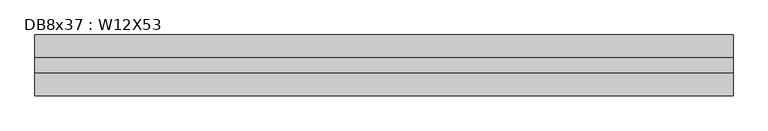
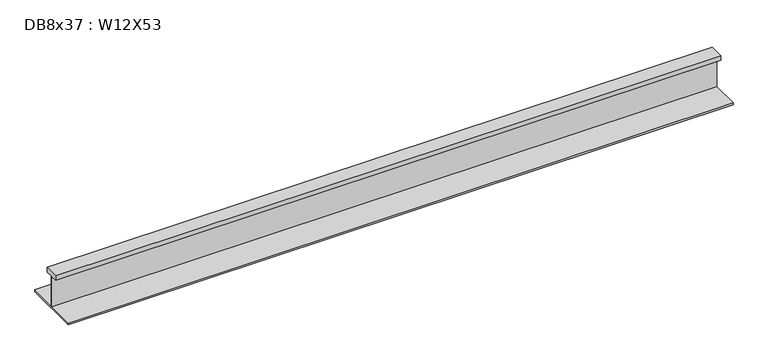
"""IFC4 building model written with IfcOpenShell, lengths in millimetres: beam geometry, DB8x37 : W12X53."""

from ifc_helpers import new_model, si_unit, frame, origin, place, context, project, spatial, polyline, outline, extrude, source, transform, mapped, element, save


def db8x37_w12x53_467f9729(model_context):
    return source(origin(), model_context, "Body", "SweptSolid", [
        extrude(outline(polyline([(38.1, 145.415), (38.1, 120.015), (2.921, 120.015), (2.921, -48.4505), (152.4, -48.4505), (152.4, -58.1025), (-152.4, -58.1025), (-152.4, -48.4505), (-2.921, -48.4505), (-2.921, 120.015), (-38.1, 120.015), (-38.1, 145.415), (38.1, 145.415)])), frame((-1711.0592287, 0.0, 0.0), z_axis=(1.0, 0.0, 0.0), x_axis=(0.0, 1.0, 0.0)), (0.0, 0.0, 1.0), 3503.6118107),
    ])


if __name__ == "__main__":
    model = new_model("IFC4")
    model_context = context("Model", 3, world=origin())
    ifc_project = project(units=[si_unit("LENGTHUNIT", "METRE", prefix="MILLI")], contexts=[model_context])
    site = spatial("IfcSite", under=ifc_project)
    building = spatial("IfcBuilding", under=site)
    placement = place(None, origin())
    db8x37_w12x53_shape = db8x37_w12x53_467f9729(model_context)
    element("IfcBeam", 1, ObjectType="DB8x37 : W12X53", at=placement, inside=building, context=model_context, shape_type="MappedRepresentation", body=[
        mapped(db8x37_w12x53_shape, transform((0.0, 0.0, 0.0), x_axis=(1.0, 0.0, 0.0), y_axis=(0.0, 1.0, 0.0), z_axis=(0.0, 0.0, 1.0))),
    ])
    save(model, "model.ifc")

# Revit data of these elements
# Type "DB8x37 : W12X53"
#   Assembly Code = "B10"
#   W = 53
#   Length [instance default] = 5' - 0"
#   bf = 0' - 10"
#   d = 1' - 0.1"
#   k = 0' - 1 3/8"
#   k2 = 0' - 0.8"
#   tf = 0' - 0.575"
#   tw = 0' - 0.345"
#   A = 0.108333 SF
#   Structural Material [instance default] = Steel ASTM A992
# Element 1 (IfcBeam, "DB8x37 : W12X53")
#   Materials on its faces: "Steel ASTM A992"
# Materials
#   "Steel ASTM A992": class "Metal", colour RGB 199 199 199, transparency 0, Description = "Structural steel 50ksi", Cost = 0
